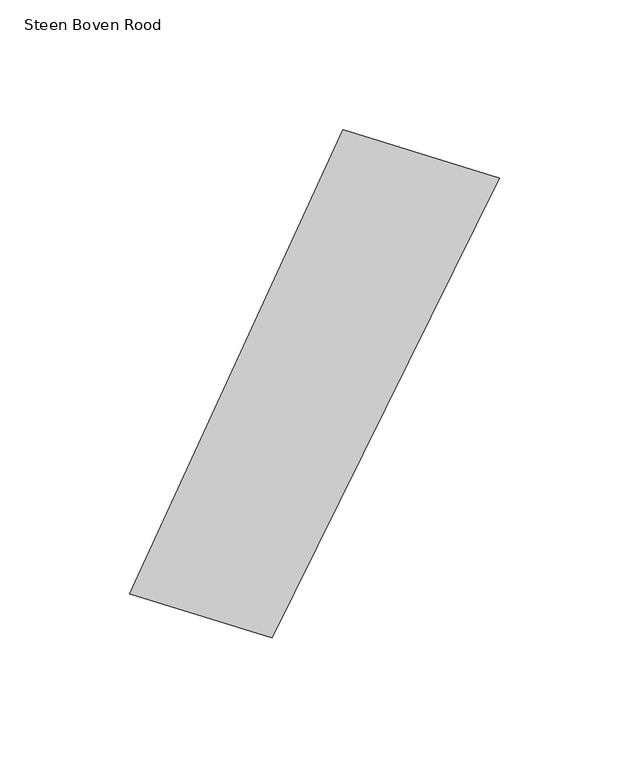
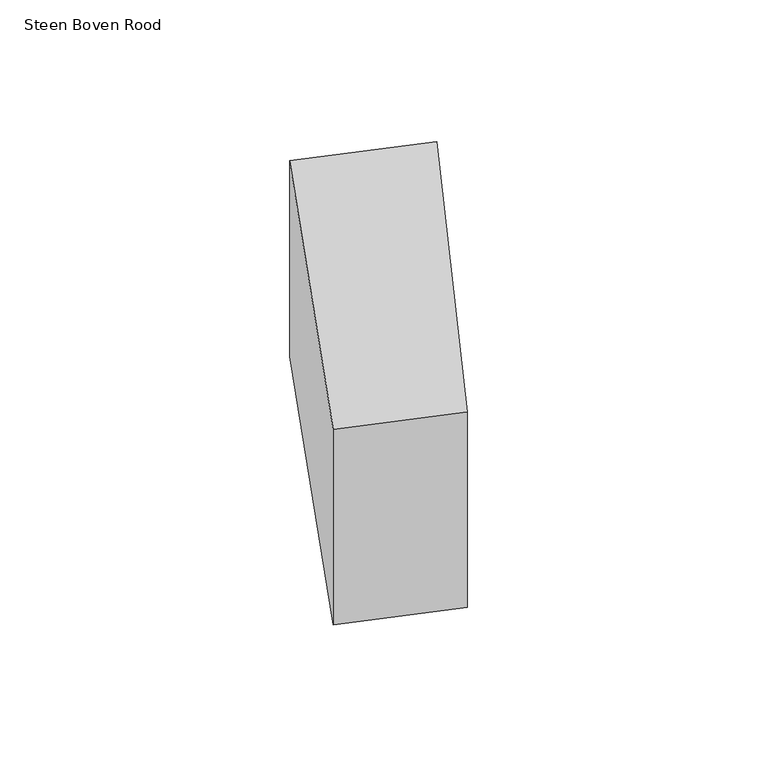
"""IFC4 building model written with IfcOpenShell, lengths in millimetres: proxy geometry, 00_GMA_steen_versie_4 : Steen Boven Rood."""

from ifc_helpers import new_model, si_unit, origin, origin_with_axes, place, context, project, spatial, polyline, outline, extrude, source, transform, mapped, element, save


def steen_boven_rood_09fe3221(model_context):
    return source(origin(), model_context, "Body", "SweptSolid", [
        extrude(outline(polyline([(145.6801741, 160.8596095), (58.0896733, -16.2293318), (3.2836628, 0.7379307), (85.4190403, 179.4954346), (145.6801741, 160.8596095)])), origin_with_axes(), (0.0, 0.0, 1.0), 100.0),
    ])


if __name__ == "__main__":
    model = new_model("IFC4")
    model_context = context("Model", 3, world=origin())
    ifc_project = project(units=[si_unit("LENGTHUNIT", "METRE", prefix="MILLI")], contexts=[model_context])
    site = spatial("IfcSite", under=ifc_project)
    building = spatial("IfcBuilding", under=site)
    placement = place(None, origin())
    steen_boven_rood_shape = steen_boven_rood_09fe3221(model_context)
    element("IfcBuildingElementProxy", 1, Name="00_GMA_steen_versie_4 : Steen Boven Rood", ObjectType="00_GMA_steen_versie_4 : Steen Boven Rood", at=placement, inside=building, context=model_context, shape_type="MappedRepresentation", body=[
        mapped(steen_boven_rood_shape, transform((0.0, 0.0, 0.0), x_axis=(1.0, 0.0, 0.0), y_axis=(0.0, 1.0, 0.0), z_axis=(0.0, 0.0, 1.0))),
    ])
    save(model, "model.ifc")

# Revit data of these elements
# Type "00_GMA_steen_versie_4 : Steen Boven Rood"
#   StootVoegHalfBoven [instance default] = 5 mm
#   StootVoegHalf [instance default] = 5 mm
#   StootVoegBreedteOnder = 10 mm
#   StootVoegBreedteBoven = 10 mm
#   Steendikte = 100 mm
#   LintVoegOnderHalf = 5 mm
#   LintVoegOnder = 10 mm
#   LintVoegBovenHalf = 0 mm
#   LintVoegBoven = 0 mm
#   materiaal = 21_steen_rood
#   MateriaalVoeg = none
#   Default Elevation = 0
# Element 1 (IfcBuildingElementProxy, "00_GMA_steen_versie_4 : Steen Boven Rood")
#   Materials on its faces: "21_steen_rood"
# Materials
#   "21_steen_rood": class "Unassigned", colour RGB 213 111 43, transparency 0, Cost = 0
